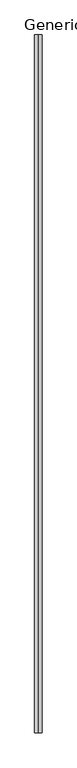
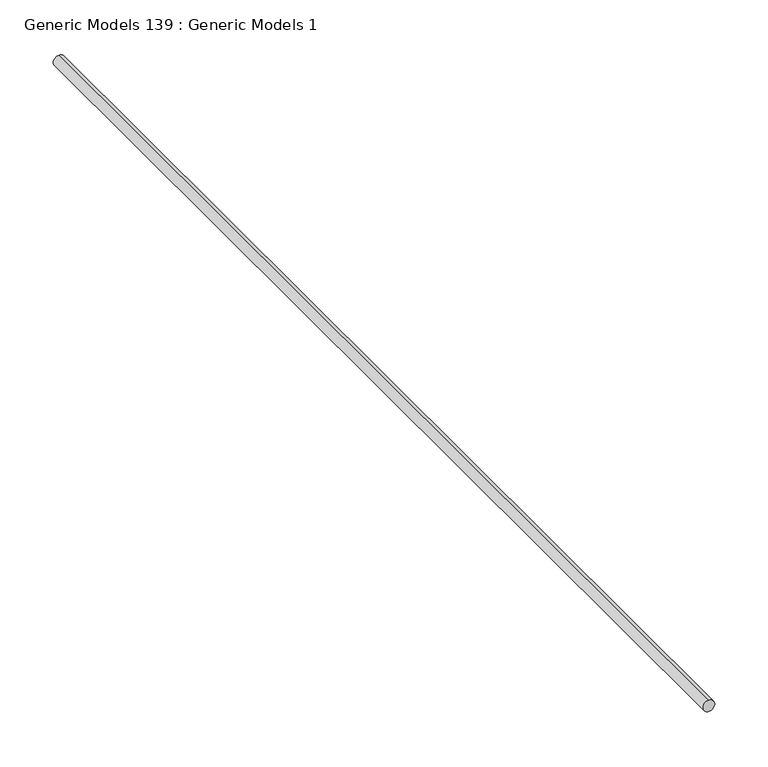
"""IFC4 building model written with IfcOpenShell, lengths in millimetres: proxy geometry, Generic Models 139 : Generic Models 1."""

import ifcopenshell
import ifcopenshell.guid

model = None  # the IFC model being written
_history = None  # IfcOwnerHistory: only IFC2X3 demands one
_inside = {}  # id of a spatial element -> (the spatial element, [elements in it])
_under = {}  # id of a project, library or spatial element -> (it, [spatial elements below it])
_declared = {}  # id of a project -> (the project, [libraries it declares])
_typed = {}  # id of a type object -> (the type object, [elements of that type])
_made_of = {}  # id of a material, layer set ... -> (it, [elements and type objects made of it])


def new_model(schema):
    """Start an empty IFC model of exactly this schema.

    Asked for "IFC4X3", IfcOpenShell would pick the latest addendum, in which some entities
    have other attributes; the version numbers below select the first issue.
    IFC2X3 requires an IfcOwnerHistory on every rooted entity: one is made here for all.
    """
    global model, _history
    if schema == "IFC4X3":
        model = ifcopenshell.file(schema_version=(4, 3, 0, 0))
    else:
        model = ifcopenshell.file(schema=schema)
    _inside.clear()
    _under.clear()
    _declared.clear()
    _typed.clear()
    _made_of.clear()
    _history = None
    if model.schema == "IFC2X3":
        org = make("IfcOrganization", Name="unknown")
        user = make(
            "IfcPersonAndOrganization",
            ThePerson=make("IfcPerson", FamilyName="unknown"),
            TheOrganization=org,
        )
        app = make(
            "IfcApplication",
            ApplicationDeveloper=org,
            Version="unknown",
            ApplicationFullName="unknown",
            ApplicationIdentifier="unknown",
        )
        _history = make(
            "IfcOwnerHistory",
            OwningUser=user,
            OwningApplication=app,
            ChangeAction="ADDED",
            CreationDate=0,
        )
    return model


def make(cls, **values):
    """One entity of the class cls with the attributes given. An attribute that is None is left unset."""
    return model.create_entity(
        cls, **{name: value for name, value in values.items() if value is not None}
    )


def rooted(cls, **values):
    """An entity with a GlobalId (a new one), such as an element, a storey or a relation."""
    return make(cls, GlobalId=ifcopenshell.guid.new(), OwnerHistory=_history, **values)


def si_unit(unit_type, name, prefix=None):
    """IfcSIUnit, for example si_unit("LENGTHUNIT", "METRE", prefix="MILLI")."""
    return make("IfcSIUnit", UnitType=unit_type, Prefix=prefix, Name=name)


def assignment(units):
    """IfcUnitAssignment: the units of a project."""
    return None if units is None else make("IfcUnitAssignment", Units=units)


def point(xyz):
    """IfcCartesianPoint."""
    return None if xyz is None else make("IfcCartesianPoint", Coordinates=xyz)


def direction(xyz):
    """IfcDirection."""
    return None if xyz is None else make("IfcDirection", DirectionRatios=xyz)


def frame(location, z_axis=None, x_axis=None):
    """IfcAxis2Placement3D, a coordinate frame: its origin and axes. An axis left out is left unset."""
    return make(
        "IfcAxis2Placement3D",
        Location=point(location),
        Axis=direction(z_axis),
        RefDirection=direction(x_axis),
    )


def frame_2d(location, x_axis=None):
    """IfcAxis2Placement2D, a coordinate frame in the plane: its origin and x axis."""
    return make(
        "IfcAxis2Placement2D", Location=point(location), RefDirection=direction(x_axis)
    )


def origin():
    """The frame at (0, 0, 0) with its axes left unset."""
    return frame((0.0, 0.0, 0.0))


def place(relative_to, where):
    """IfcLocalPlacement: puts the frame where relative to a parent placement (None: the world)."""
    return make(
        "IfcLocalPlacement", PlacementRelTo=relative_to, RelativePlacement=where
    )


def context(
    kind, dimensions, precision=None, world=None, true_north=None, identifier=None
):
    """IfcGeometricRepresentationContext, for example the 3D "Model" context."""
    return make(
        "IfcGeometricRepresentationContext",
        ContextIdentifier=identifier,
        ContextType=kind,
        CoordinateSpaceDimension=dimensions,
        Precision=precision,
        WorldCoordinateSystem=world,
        TrueNorth=true_north,
    )


def project(units=None, contexts=None):
    """IfcProject with its units and contexts."""
    return rooted(
        "IfcProject",
        Name="project",
        RepresentationContexts=contexts,
        UnitsInContext=assignment(units),
    )


def spatial(cls, under=None, at=None, **own):
    """A site, building, storey or space (cls), placed at a placement, below another one or the project."""
    s = rooted(cls, ObjectPlacement=at, **own)
    if under is not None:
        _under.setdefault(under.id(), (under, []))[1].append(s)
    return s


def circle_curve(where, radius):
    """IfcCircle in the frame where."""
    return make("IfcCircle", Position=where, Radius=radius)


def trimmed(basis, trim1, trim2, sense, master):
    """IfcTrimmedCurve: the piece of a basis curve between two trims."""
    return make(
        "IfcTrimmedCurve",
        BasisCurve=basis,
        Trim1=trim1,
        Trim2=trim2,
        SenseAgreement=sense,
        MasterRepresentation=master,
    )


def segment(curve, same_sense, transition):
    """IfcCompositeCurveSegment."""
    return make(
        "IfcCompositeCurveSegment",
        Transition=transition,
        SameSense=same_sense,
        ParentCurve=curve,
    )


def composite_curve(segments, self_intersect=None):
    """IfcCompositeCurve: segments joined end to end."""
    return make("IfcCompositeCurve", Segments=segments, SelfIntersect=self_intersect)


def outline(outer, holes=None, kind="AREA"):
    """IfcArbitraryClosedProfileDef: a profile drawn as a closed curve; with holes, ...WithVoids."""
    if holes is None:
        return make("IfcArbitraryClosedProfileDef", ProfileType=kind, OuterCurve=outer)
    return make(
        "IfcArbitraryProfileDefWithVoids",
        ProfileType=kind,
        OuterCurve=outer,
        InnerCurves=holes,
    )


def extrude(swept, where, along, depth):
    """IfcExtrudedAreaSolid: the profile swept, set in the frame where, extruded along a direction by depth."""
    return make(
        "IfcExtrudedAreaSolid",
        SweptArea=swept,
        Position=where,
        ExtrudedDirection=direction(along),
        Depth=depth,
    )


def shape(context_of_items, identifier, shape_type, items):
    """IfcShapeRepresentation: the items that make up one representation, for example the "Body"."""
    return make(
        "IfcShapeRepresentation",
        ContextOfItems=context_of_items,
        RepresentationIdentifier=identifier,
        RepresentationType=shape_type,
        Items=items,
    )


def source(mapping_origin, context_of_items, identifier, shape_type, items):
    """IfcRepresentationMap: a shape defined once, which mapped items show again and again."""
    return make(
        "IfcRepresentationMap",
        MappingOrigin=mapping_origin,
        MappedRepresentation=shape(context_of_items, identifier, shape_type, items),
    )


def transform(
    local_origin,
    x_axis=None,
    y_axis=None,
    z_axis=None,
    scale=None,
    scale2=None,
    scale3=None,
    uniform=True,
):
    """IfcCartesianTransformationOperator3D, or its non-uniform kind. x_axis, y_axis, z_axis: its Axis1, 2, 3."""
    if uniform:
        return make(
            "IfcCartesianTransformationOperator3D",
            Axis1=direction(x_axis),
            Axis2=direction(y_axis),
            LocalOrigin=point(local_origin),
            Scale=scale,
            Axis3=direction(z_axis),
        )
    return make(
        "IfcCartesianTransformationOperator3DnonUniform",
        Axis1=direction(x_axis),
        Axis2=direction(y_axis),
        LocalOrigin=point(local_origin),
        Scale=scale,
        Axis3=direction(z_axis),
        Scale2=scale2,
        Scale3=scale3,
    )


def mapped(mapping_source, mapping_target):
    """IfcMappedItem: shows the shape of a source again, moved by a transform."""
    return make(
        "IfcMappedItem", MappingSource=mapping_source, MappingTarget=mapping_target
    )


def made_of(thing, what):
    """Note that an element or type object is made of a material, layer set ...; save() writes the relation."""
    if what is not None:
        _made_of.setdefault(what.id(), (what, []))[1].append(thing)
    return thing


def element(
    cls,
    number,
    at=None,
    inside=None,
    cuts=None,
    type_object=None,
    material=None,
    context=None,
    identifier="Body",
    shape_type=None,
    held_by="IfcProductDefinitionShape",
    body=None,
    shapes=None,
    **own,
):
    """One element of the class cls, such as IfcWall. Its Tag is "e" and its number.

    at: its placement. inside: the storey or other place that contains it. cuts: it is an
    opening in that element (IfcRelVoidsElement). A single representation is given by context,
    identifier, shape_type and body (its items); several are given by shapes. held_by: the class
    of the entity that holds the representations. save() writes the other relations.
    """
    e = rooted(cls, Tag="e%d" % number, ObjectPlacement=at, **own)
    if body is not None:
        shapes = [shape(context, identifier, shape_type, body)]
    if shapes is not None:
        e.Representation = make(held_by, Representations=shapes)
    if inside is not None:
        _inside.setdefault(inside.id(), (inside, []))[1].append(e)
    if cuts is not None:
        rooted(
            "IfcRelVoidsElement", RelatingBuildingElement=cuts, RelatedOpeningElement=e
        )
    if type_object is not None:
        _typed.setdefault(type_object.id(), (type_object, []))[1].append(e)
    return made_of(e, material)


def aggregate(whole, parts):
    """IfcRelAggregates: a whole, such as a stair, and the parts it consists of."""
    return rooted("IfcRelAggregates", RelatingObject=whole, RelatedObjects=parts)


def save(model, path):
    """Write the relations noted so far, then the file.

    IfcRelAggregates (storeys below a building ...), IfcRelContainedInSpatialStructure (elements
    in a storey), IfcRelDefinesByType, IfcRelAssociatesMaterial and IfcRelDeclares: one each for
    every whole, place, type object, material and project.
    """
    for whole, parts in _under.values():
        aggregate(whole, parts)
    for where, things in _inside.values():
        rooted(
            "IfcRelContainedInSpatialStructure",
            RelatedElements=things,
            RelatingStructure=where,
        )
    for kind, things in _typed.values():
        rooted("IfcRelDefinesByType", RelatedObjects=things, RelatingType=kind)
    for what, things in _made_of.values():
        rooted("IfcRelAssociatesMaterial", RelatedObjects=things, RelatingMaterial=what)
    for by, libraries in _declared.values():
        rooted("IfcRelDeclares", RelatingContext=by, RelatedDefinitions=libraries)
    model.write(path)


def generic_models_139_generic_models_1_e596f594(model_context):
    return source(origin(), model_context, "Body", "SweptSolid", [
        extrude(outline(composite_curve([segment(trimmed(circle_curve(frame_2d((97.5288266, 52112.9548165)), 6.35), [point((91.1788266, 52112.9548165))], [point((103.8788266, 52112.9548165))], False, "CARTESIAN"), True, "CONTINUOUS"), segment(trimmed(circle_curve(frame_2d((97.5288266, 52112.9548165)), 6.35), [point((103.8788266, 52112.9548165))], [point((91.1788266, 52112.9548165))], False, "CARTESIAN"), True, "CONTINUOUS")], self_intersect=False)), frame((0.0, 0.0, 0.0), z_axis=(0.0, 1.0, 0.0), x_axis=(0.0, 0.0, 1.0)), (0.0, 0.0, 1.0), 1219.2),
    ])


if __name__ == "__main__":
    model = new_model("IFC4")
    model_context = context("Model", 3, world=origin())
    ifc_project = project(units=[si_unit("LENGTHUNIT", "METRE", prefix="MILLI")], contexts=[model_context])
    site = spatial("IfcSite", under=ifc_project)
    building = spatial("IfcBuilding", under=site)
    placement = place(None, origin())
    generic_models_139_generic_models_1_shape = generic_models_139_generic_models_1_e596f594(model_context)
    element("IfcBuildingElementProxy", 1, Name="Generic Models 139 : Generic Models 1", ObjectType="Generic Models 139 : Generic Models 1", at=placement, inside=building, context=model_context, shape_type="MappedRepresentation", body=[
        mapped(generic_models_139_generic_models_1_shape, transform((0.0, 0.0, 0.0), x_axis=(1.0, 0.0, 0.0), y_axis=(0.0, 1.0, 0.0), z_axis=(0.0, 0.0, 1.0))),
    ])
    save(model, "model.ifc")

# Revit data of these elements
# Element 1 (IfcBuildingElementProxy, "Generic Models 139 : Generic Models 1")
#   Materials on its faces: "#4 CONT. STEEL REBAR"
# Materials
#   "#4 CONT. STEEL REBAR": class "Metal", colour RGB 189 187 185, transparency 0, Description = "Structural steel 50ksi", Cost = 0
